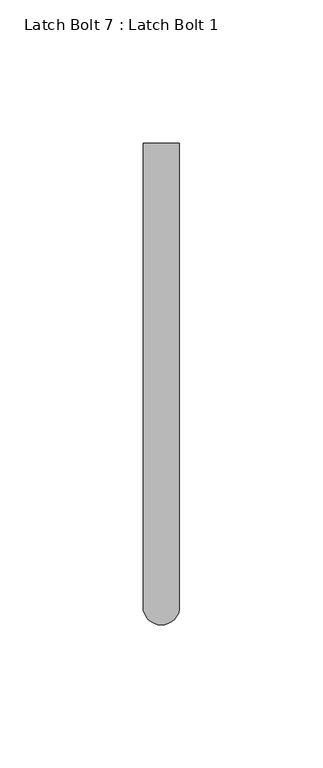
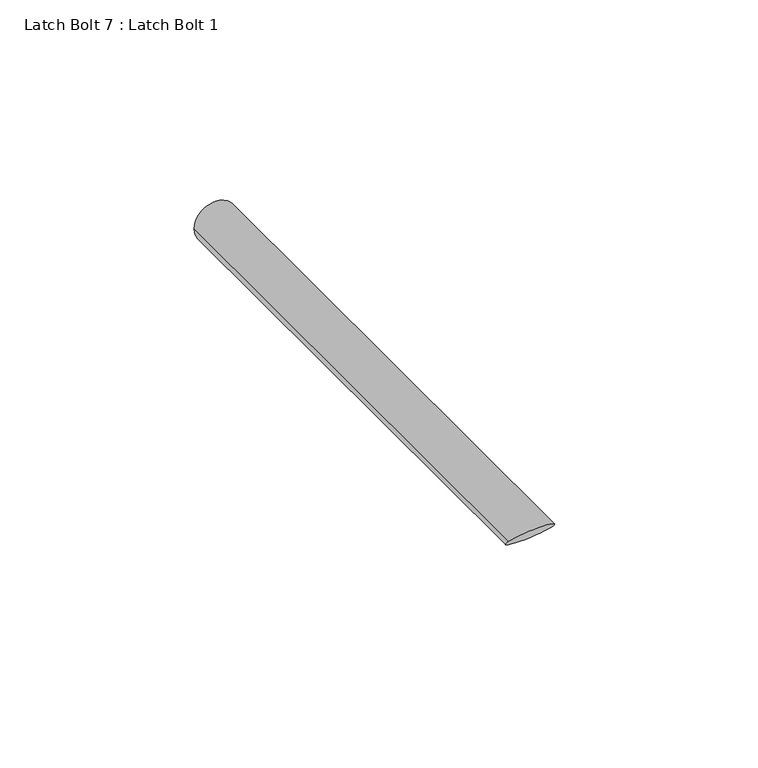
"""IFC4 building model written with IfcOpenShell, lengths in millimetres: proxy geometry, Latch Bolt 7 : Latch Bolt 1."""

import ifcopenshell
import ifcopenshell.guid

model = None  # the IFC model being written
_history = None  # IfcOwnerHistory: only IFC2X3 demands one
_inside = {}  # id of a spatial element -> (the spatial element, [elements in it])
_under = {}  # id of a project, library or spatial element -> (it, [spatial elements below it])
_declared = {}  # id of a project -> (the project, [libraries it declares])
_typed = {}  # id of a type object -> (the type object, [elements of that type])
_made_of = {}  # id of a material, layer set ... -> (it, [elements and type objects made of it])


def new_model(schema):
    """Start an empty IFC model of exactly this schema.

    Asked for "IFC4X3", IfcOpenShell would pick the latest addendum, in which some entities
    have other attributes; the version numbers below select the first issue.
    IFC2X3 requires an IfcOwnerHistory on every rooted entity: one is made here for all.
    """
    global model, _history
    if schema == "IFC4X3":
        model = ifcopenshell.file(schema_version=(4, 3, 0, 0))
    else:
        model = ifcopenshell.file(schema=schema)
    _inside.clear()
    _under.clear()
    _declared.clear()
    _typed.clear()
    _made_of.clear()
    _history = None
    if model.schema == "IFC2X3":
        org = make("IfcOrganization", Name="unknown")
        user = make(
            "IfcPersonAndOrganization",
            ThePerson=make("IfcPerson", FamilyName="unknown"),
            TheOrganization=org,
        )
        app = make(
            "IfcApplication",
            ApplicationDeveloper=org,
            Version="unknown",
            ApplicationFullName="unknown",
            ApplicationIdentifier="unknown",
        )
        _history = make(
            "IfcOwnerHistory",
            OwningUser=user,
            OwningApplication=app,
            ChangeAction="ADDED",
            CreationDate=0,
        )
    return model


def make(cls, **values):
    """One entity of the class cls with the attributes given. An attribute that is None is left unset."""
    return model.create_entity(
        cls, **{name: value for name, value in values.items() if value is not None}
    )


def rooted(cls, **values):
    """An entity with a GlobalId (a new one), such as an element, a storey or a relation."""
    return make(cls, GlobalId=ifcopenshell.guid.new(), OwnerHistory=_history, **values)


def si_unit(unit_type, name, prefix=None):
    """IfcSIUnit, for example si_unit("LENGTHUNIT", "METRE", prefix="MILLI")."""
    return make("IfcSIUnit", UnitType=unit_type, Prefix=prefix, Name=name)


def assignment(units):
    """IfcUnitAssignment: the units of a project."""
    return None if units is None else make("IfcUnitAssignment", Units=units)


def point(xyz):
    """IfcCartesianPoint."""
    return None if xyz is None else make("IfcCartesianPoint", Coordinates=xyz)


def direction(xyz):
    """IfcDirection."""
    return None if xyz is None else make("IfcDirection", DirectionRatios=xyz)


def frame(location, z_axis=None, x_axis=None):
    """IfcAxis2Placement3D, a coordinate frame: its origin and axes. An axis left out is left unset."""
    return make(
        "IfcAxis2Placement3D",
        Location=point(location),
        Axis=direction(z_axis),
        RefDirection=direction(x_axis),
    )


def origin():
    """The frame at (0, 0, 0) with its axes left unset."""
    return frame((0.0, 0.0, 0.0))


def place(relative_to, where):
    """IfcLocalPlacement: puts the frame where relative to a parent placement (None: the world)."""
    return make(
        "IfcLocalPlacement", PlacementRelTo=relative_to, RelativePlacement=where
    )


def context(
    kind, dimensions, precision=None, world=None, true_north=None, identifier=None
):
    """IfcGeometricRepresentationContext, for example the 3D "Model" context."""
    return make(
        "IfcGeometricRepresentationContext",
        ContextIdentifier=identifier,
        ContextType=kind,
        CoordinateSpaceDimension=dimensions,
        Precision=precision,
        WorldCoordinateSystem=world,
        TrueNorth=true_north,
    )


def project(units=None, contexts=None):
    """IfcProject with its units and contexts."""
    return rooted(
        "IfcProject",
        Name="project",
        RepresentationContexts=contexts,
        UnitsInContext=assignment(units),
    )


def spatial(cls, under=None, at=None, **own):
    """A site, building, storey or space (cls), placed at a placement, below another one or the project."""
    s = rooted(cls, ObjectPlacement=at, **own)
    if under is not None:
        _under.setdefault(under.id(), (under, []))[1].append(s)
    return s


def circle_curve(where, radius):
    """IfcCircle in the frame where."""
    return make("IfcCircle", Position=where, Radius=radius)


def ellipse_curve(where, semi_axis1, semi_axis2):
    """IfcEllipse in the frame where."""
    return make(
        "IfcEllipse", Position=where, SemiAxis1=semi_axis1, SemiAxis2=semi_axis2
    )


def shape(context_of_items, identifier, shape_type, items):
    """IfcShapeRepresentation: the items that make up one representation, for example the "Body"."""
    return make(
        "IfcShapeRepresentation",
        ContextOfItems=context_of_items,
        RepresentationIdentifier=identifier,
        RepresentationType=shape_type,
        Items=items,
    )


def source(mapping_origin, context_of_items, identifier, shape_type, items):
    """IfcRepresentationMap: a shape defined once, which mapped items show again and again."""
    return make(
        "IfcRepresentationMap",
        MappingOrigin=mapping_origin,
        MappedRepresentation=shape(context_of_items, identifier, shape_type, items),
    )


def transform(
    local_origin,
    x_axis=None,
    y_axis=None,
    z_axis=None,
    scale=None,
    scale2=None,
    scale3=None,
    uniform=True,
):
    """IfcCartesianTransformationOperator3D, or its non-uniform kind. x_axis, y_axis, z_axis: its Axis1, 2, 3."""
    if uniform:
        return make(
            "IfcCartesianTransformationOperator3D",
            Axis1=direction(x_axis),
            Axis2=direction(y_axis),
            LocalOrigin=point(local_origin),
            Scale=scale,
            Axis3=direction(z_axis),
        )
    return make(
        "IfcCartesianTransformationOperator3DnonUniform",
        Axis1=direction(x_axis),
        Axis2=direction(y_axis),
        LocalOrigin=point(local_origin),
        Scale=scale,
        Axis3=direction(z_axis),
        Scale2=scale2,
        Scale3=scale3,
    )


def mapped(mapping_source, mapping_target):
    """IfcMappedItem: shows the shape of a source again, moved by a transform."""
    return make(
        "IfcMappedItem", MappingSource=mapping_source, MappingTarget=mapping_target
    )


def made_of(thing, what):
    """Note that an element or type object is made of a material, layer set ...; save() writes the relation."""
    if what is not None:
        _made_of.setdefault(what.id(), (what, []))[1].append(thing)
    return thing


def element(
    cls,
    number,
    at=None,
    inside=None,
    cuts=None,
    type_object=None,
    material=None,
    context=None,
    identifier="Body",
    shape_type=None,
    held_by="IfcProductDefinitionShape",
    body=None,
    shapes=None,
    **own,
):
    """One element of the class cls, such as IfcWall. Its Tag is "e" and its number.

    at: its placement. inside: the storey or other place that contains it. cuts: it is an
    opening in that element (IfcRelVoidsElement). A single representation is given by context,
    identifier, shape_type and body (its items); several are given by shapes. held_by: the class
    of the entity that holds the representations. save() writes the other relations.
    """
    e = rooted(cls, Tag="e%d" % number, ObjectPlacement=at, **own)
    if body is not None:
        shapes = [shape(context, identifier, shape_type, body)]
    if shapes is not None:
        e.Representation = make(held_by, Representations=shapes)
    if inside is not None:
        _inside.setdefault(inside.id(), (inside, []))[1].append(e)
    if cuts is not None:
        rooted(
            "IfcRelVoidsElement", RelatingBuildingElement=cuts, RelatedOpeningElement=e
        )
    if type_object is not None:
        _typed.setdefault(type_object.id(), (type_object, []))[1].append(e)
    return made_of(e, material)


def aggregate(whole, parts):
    """IfcRelAggregates: a whole, such as a stair, and the parts it consists of."""
    return rooted("IfcRelAggregates", RelatingObject=whole, RelatedObjects=parts)


def save(model, path):
    """Write the relations noted so far, then the file.

    IfcRelAggregates (storeys below a building ...), IfcRelContainedInSpatialStructure (elements
    in a storey), IfcRelDefinesByType, IfcRelAssociatesMaterial and IfcRelDeclares: one each for
    every whole, place, type object, material and project.
    """
    for whole, parts in _under.values():
        aggregate(whole, parts)
    for where, things in _inside.values():
        rooted(
            "IfcRelContainedInSpatialStructure",
            RelatedElements=things,
            RelatingStructure=where,
        )
    for kind, things in _typed.values():
        rooted("IfcRelDefinesByType", RelatedObjects=things, RelatingType=kind)
    for what, things in _made_of.values():
        rooted("IfcRelAssociatesMaterial", RelatedObjects=things, RelatingMaterial=what)
    for by, libraries in _declared.values():
        rooted("IfcRelDeclares", RelatingContext=by, RelatedDefinitions=libraries)
    model.write(path)


def plane_surface(at):
    """IfcPlane: the flat surface through the origin of the frame at, square to its z axis."""
    return make("IfcPlane", Position=at)


def cylinder_surface(at, radius):
    """IfcCylindricalSurface: all points at the distance radius from the z axis of the frame at."""
    return make("IfcCylindricalSurface", Position=at, Radius=radius)


def advanced_brep(points, edges, surfaces, faces):
    """IfcAdvancedBrep: a solid bounded by faces that lie on surfaces and meet in shared edges.

    An edge is (start, end): straight between two places in points (the first is 0);
    or (start, end, curve); or (start, end, curve, False) where it runs against its curve.
    A face is (place in surfaces, loops), or (place, loops, False) where it looks against
    its surface's normal. A loop lists edges by number (the first is 1), with a minus sign
    where the edge is run from its end to its start. The first loop is the outer one.
    """
    corners = [point(p) for p in points]
    vertices = [make("IfcVertexPoint", VertexGeometry=c) for c in corners]
    made = []
    for start, end, *more in edges:
        made.append(
            make(
                "IfcEdgeCurve",
                EdgeStart=vertices[start],
                EdgeEnd=vertices[end],
                EdgeGeometry=more[0] if more else make("IfcPolyline", Points=[corners[start], corners[end]]),
                SameSense=more[1] if len(more) > 1 else True,
            )
        )
    hull = []
    for where, loops, *sense in faces:
        bounds = []
        for j, loop in enumerate(loops):
            ring = [make("IfcOrientedEdge", EdgeElement=made[abs(k) - 1], Orientation=k > 0) for k in loop]
            bounds.append(
                make(
                    "IfcFaceOuterBound" if j == 0 else "IfcFaceBound",
                    Bound=make("IfcEdgeLoop", EdgeList=ring),
                    Orientation=True,
                )
            )
        hull.append(make("IfcAdvancedFace", Bounds=bounds, FaceSurface=surfaces[where], SameSense=sense[0] if sense else True))
    return make("IfcAdvancedBrep", Outer=make("IfcClosedShell", CfsFaces=hull))


def latch_bolt_7_latch_bolt_1_d9de4a67(model_context):
    return source(origin(), model_context, "Body", "AdvancedBrep", [
        advanced_brep(
        [(587306.3685739, -532807.6163841, 1066.8), (587319.0685739, -532807.6163841, 1066.8), (587306.3685739, -532969.5413841, 1066.8), (587312.7185739, -532975.8913841, 1073.15), (587319.0685739, -532969.5413841, 1066.8)],
        [
            (0, 1, circle_curve(frame((587312.7185739, -532807.6163841, 1066.8), z_axis=(0.0, 1.0, 0.0), x_axis=(1.0, 0.0, 0.0)), 6.35)),
            (1, 0, circle_curve(frame((587312.7185739, -532807.6163841, 1066.8), z_axis=(0.0, 1.0, 0.0), x_axis=(1.0, 0.0, 0.0)), 6.35)),
            (0, 2),
            (2, 3, ellipse_curve(frame((587312.7185739, -532969.5413841, 1066.8), z_axis=(0.0, 0.7071067811870104, 0.7071067811860847), x_axis=(0.0, 0.7071067811860846, -0.7071067811870104)), 8.9802561, 6.35)),
            (3, 4, ellipse_curve(frame((587312.7185739, -532969.5413841, 1066.8), z_axis=(0.0, 0.7071067811870104, 0.7071067811860847), x_axis=(0.0, 0.7071067811860846, -0.7071067811870104)), 8.9802561, 6.35)),
            (4, 1),
            (4, 2, ellipse_curve(frame((587312.7185739, -532969.5413841, 1066.8), z_axis=(0.0, 0.7071067811870104, 0.7071067811860847), x_axis=(0.0, 0.7071067811860846, -0.7071067811870104)), 8.9802561, 6.35)),
        ],
        [
            plane_surface(frame((587319.0685739, -532807.6163841, 1066.8), z_axis=(0.0, 1.0, 0.0), x_axis=(0.0, 0.0, -1.0))),
            cylinder_surface(frame((587312.7185739, -532975.8913841, 1066.8), z_axis=(0.0, 1.0, 0.0), x_axis=(1.0, 0.0, 0.0)), 6.35),
            plane_surface(frame((587338.1185739, -532960.0163841, 1057.275), z_axis=(0.0, -0.7071067811870104, -0.7071067811860847), x_axis=(-1.0, 0.0, 0.0))),
        ],
        [
            (0, [[1, 2]]),
            (1, [[-1, 3, 4, 5, 6]]),
            (1, [[-2, -6, 7, -3]]),
            (2, [[-4, -7, -5]]),
        ],
    ),
    ])


if __name__ == "__main__":
    model = new_model("IFC4")
    model_context = context("Model", 3, world=origin())
    ifc_project = project(units=[si_unit("LENGTHUNIT", "METRE", prefix="MILLI")], contexts=[model_context])
    site = spatial("IfcSite", under=ifc_project)
    building = spatial("IfcBuilding", under=site)
    placement = place(None, origin())
    latch_bolt_7_latch_bolt_1_shape = latch_bolt_7_latch_bolt_1_d9de4a67(model_context)
    element("IfcBuildingElementProxy", 1, Name="Latch Bolt 7 : Latch Bolt 1", ObjectType="Latch Bolt 7 : Latch Bolt 1", at=placement, inside=building, context=model_context, shape_type="MappedRepresentation", body=[
        mapped(latch_bolt_7_latch_bolt_1_shape, transform((0.0, 0.0, 0.0), x_axis=(1.0, 0.0, 0.0), y_axis=(0.0, 1.0, 0.0), z_axis=(0.0, 0.0, 1.0))),
    ])
    save(model, "model.ifc")

# Revit data of these elements
# Element 1 (IfcBuildingElementProxy, "Latch Bolt 7 : Latch Bolt 1")
#   Materials on its faces: "GALV. GATE LATCH"
# Materials
#   "GALV. GATE LATCH": class "Metal", colour RGB 189 187 185, transparency 0, Description = "Carbon steel", Cost = 0
